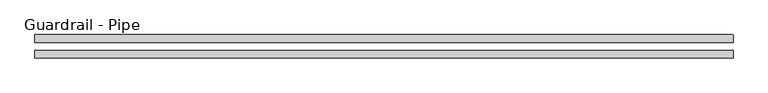
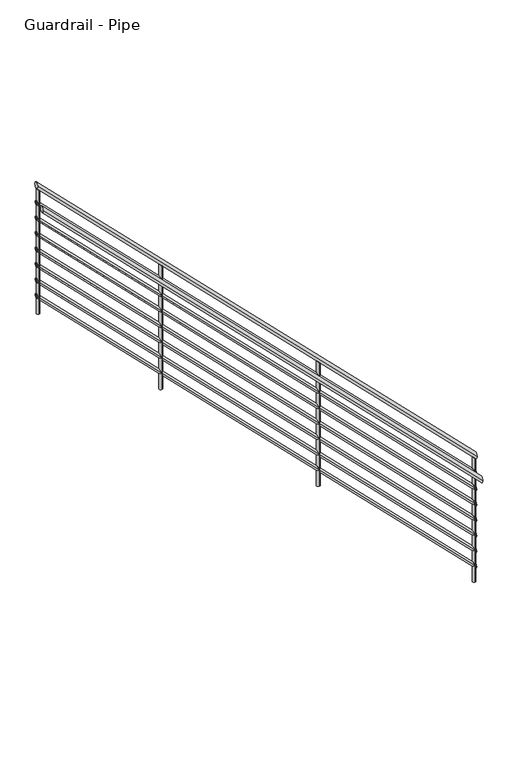
"""IFC4 building model written with IfcOpenShell, lengths in millimetres: railing geometry, Guardrail - Pipe."""

import ifcopenshell
import ifcopenshell.guid

model = None  # the IFC model being written
_history = None  # IfcOwnerHistory: only IFC2X3 demands one
_inside = {}  # id of a spatial element -> (the spatial element, [elements in it])
_under = {}  # id of a project, library or spatial element -> (it, [spatial elements below it])
_declared = {}  # id of a project -> (the project, [libraries it declares])
_typed = {}  # id of a type object -> (the type object, [elements of that type])
_made_of = {}  # id of a material, layer set ... -> (it, [elements and type objects made of it])


def new_model(schema):
    """Start an empty IFC model of exactly this schema.

    Asked for "IFC4X3", IfcOpenShell would pick the latest addendum, in which some entities
    have other attributes; the version numbers below select the first issue.
    IFC2X3 requires an IfcOwnerHistory on every rooted entity: one is made here for all.
    """
    global model, _history
    if schema == "IFC4X3":
        model = ifcopenshell.file(schema_version=(4, 3, 0, 0))
    else:
        model = ifcopenshell.file(schema=schema)
    _inside.clear()
    _under.clear()
    _declared.clear()
    _typed.clear()
    _made_of.clear()
    _history = None
    if model.schema == "IFC2X3":
        org = make("IfcOrganization", Name="unknown")
        user = make(
            "IfcPersonAndOrganization",
            ThePerson=make("IfcPerson", FamilyName="unknown"),
            TheOrganization=org,
        )
        app = make(
            "IfcApplication",
            ApplicationDeveloper=org,
            Version="unknown",
            ApplicationFullName="unknown",
            ApplicationIdentifier="unknown",
        )
        _history = make(
            "IfcOwnerHistory",
            OwningUser=user,
            OwningApplication=app,
            ChangeAction="ADDED",
            CreationDate=0,
        )
    return model


def make(cls, **values):
    """One entity of the class cls with the attributes given. An attribute that is None is left unset."""
    return model.create_entity(
        cls, **{name: value for name, value in values.items() if value is not None}
    )


def rooted(cls, **values):
    """An entity with a GlobalId (a new one), such as an element, a storey or a relation."""
    return make(cls, GlobalId=ifcopenshell.guid.new(), OwnerHistory=_history, **values)


def si_unit(unit_type, name, prefix=None):
    """IfcSIUnit, for example si_unit("LENGTHUNIT", "METRE", prefix="MILLI")."""
    return make("IfcSIUnit", UnitType=unit_type, Prefix=prefix, Name=name)


def assignment(units):
    """IfcUnitAssignment: the units of a project."""
    return None if units is None else make("IfcUnitAssignment", Units=units)


def point(xyz):
    """IfcCartesianPoint."""
    return None if xyz is None else make("IfcCartesianPoint", Coordinates=xyz)


def direction(xyz):
    """IfcDirection."""
    return None if xyz is None else make("IfcDirection", DirectionRatios=xyz)


def frame(location, z_axis=None, x_axis=None):
    """IfcAxis2Placement3D, a coordinate frame: its origin and axes. An axis left out is left unset."""
    return make(
        "IfcAxis2Placement3D",
        Location=point(location),
        Axis=direction(z_axis),
        RefDirection=direction(x_axis),
    )


def origin():
    """The frame at (0, 0, 0) with its axes left unset."""
    return frame((0.0, 0.0, 0.0))


def place(relative_to, where):
    """IfcLocalPlacement: puts the frame where relative to a parent placement (None: the world)."""
    return make(
        "IfcLocalPlacement", PlacementRelTo=relative_to, RelativePlacement=where
    )


def context(
    kind, dimensions, precision=None, world=None, true_north=None, identifier=None
):
    """IfcGeometricRepresentationContext, for example the 3D "Model" context."""
    return make(
        "IfcGeometricRepresentationContext",
        ContextIdentifier=identifier,
        ContextType=kind,
        CoordinateSpaceDimension=dimensions,
        Precision=precision,
        WorldCoordinateSystem=world,
        TrueNorth=true_north,
    )


def project(units=None, contexts=None):
    """IfcProject with its units and contexts."""
    return rooted(
        "IfcProject",
        Name="project",
        RepresentationContexts=contexts,
        UnitsInContext=assignment(units),
    )


def spatial(cls, under=None, at=None, **own):
    """A site, building, storey or space (cls), placed at a placement, below another one or the project."""
    s = rooted(cls, ObjectPlacement=at, **own)
    if under is not None:
        _under.setdefault(under.id(), (under, []))[1].append(s)
    return s


def circle_curve(where, radius):
    """IfcCircle in the frame where."""
    return make("IfcCircle", Position=where, Radius=radius)


def ellipse_curve(where, semi_axis1, semi_axis2):
    """IfcEllipse in the frame where."""
    return make(
        "IfcEllipse", Position=where, SemiAxis1=semi_axis1, SemiAxis2=semi_axis2
    )


def shape(context_of_items, identifier, shape_type, items):
    """IfcShapeRepresentation: the items that make up one representation, for example the "Body"."""
    return make(
        "IfcShapeRepresentation",
        ContextOfItems=context_of_items,
        RepresentationIdentifier=identifier,
        RepresentationType=shape_type,
        Items=items,
    )


def source(mapping_origin, context_of_items, identifier, shape_type, items):
    """IfcRepresentationMap: a shape defined once, which mapped items show again and again."""
    return make(
        "IfcRepresentationMap",
        MappingOrigin=mapping_origin,
        MappedRepresentation=shape(context_of_items, identifier, shape_type, items),
    )


def transform(
    local_origin,
    x_axis=None,
    y_axis=None,
    z_axis=None,
    scale=None,
    scale2=None,
    scale3=None,
    uniform=True,
):
    """IfcCartesianTransformationOperator3D, or its non-uniform kind. x_axis, y_axis, z_axis: its Axis1, 2, 3."""
    if uniform:
        return make(
            "IfcCartesianTransformationOperator3D",
            Axis1=direction(x_axis),
            Axis2=direction(y_axis),
            LocalOrigin=point(local_origin),
            Scale=scale,
            Axis3=direction(z_axis),
        )
    return make(
        "IfcCartesianTransformationOperator3DnonUniform",
        Axis1=direction(x_axis),
        Axis2=direction(y_axis),
        LocalOrigin=point(local_origin),
        Scale=scale,
        Axis3=direction(z_axis),
        Scale2=scale2,
        Scale3=scale3,
    )


def mapped(mapping_source, mapping_target):
    """IfcMappedItem: shows the shape of a source again, moved by a transform."""
    return make(
        "IfcMappedItem", MappingSource=mapping_source, MappingTarget=mapping_target
    )


def made_of(thing, what):
    """Note that an element or type object is made of a material, layer set ...; save() writes the relation."""
    if what is not None:
        _made_of.setdefault(what.id(), (what, []))[1].append(thing)
    return thing


def element(
    cls,
    number,
    at=None,
    inside=None,
    cuts=None,
    type_object=None,
    material=None,
    context=None,
    identifier="Body",
    shape_type=None,
    held_by="IfcProductDefinitionShape",
    body=None,
    shapes=None,
    **own,
):
    """One element of the class cls, such as IfcWall. Its Tag is "e" and its number.

    at: its placement. inside: the storey or other place that contains it. cuts: it is an
    opening in that element (IfcRelVoidsElement). A single representation is given by context,
    identifier, shape_type and body (its items); several are given by shapes. held_by: the class
    of the entity that holds the representations. save() writes the other relations.
    """
    e = rooted(cls, Tag="e%d" % number, ObjectPlacement=at, **own)
    if body is not None:
        shapes = [shape(context, identifier, shape_type, body)]
    if shapes is not None:
        e.Representation = make(held_by, Representations=shapes)
    if inside is not None:
        _inside.setdefault(inside.id(), (inside, []))[1].append(e)
    if cuts is not None:
        rooted(
            "IfcRelVoidsElement", RelatingBuildingElement=cuts, RelatedOpeningElement=e
        )
    if type_object is not None:
        _typed.setdefault(type_object.id(), (type_object, []))[1].append(e)
    return made_of(e, material)


def aggregate(whole, parts):
    """IfcRelAggregates: a whole, such as a stair, and the parts it consists of."""
    return rooted("IfcRelAggregates", RelatingObject=whole, RelatedObjects=parts)


def save(model, path):
    """Write the relations noted so far, then the file.

    IfcRelAggregates (storeys below a building ...), IfcRelContainedInSpatialStructure (elements
    in a storey), IfcRelDefinesByType, IfcRelAssociatesMaterial and IfcRelDeclares: one each for
    every whole, place, type object, material and project.
    """
    for whole, parts in _under.values():
        aggregate(whole, parts)
    for where, things in _inside.values():
        rooted(
            "IfcRelContainedInSpatialStructure",
            RelatedElements=things,
            RelatingStructure=where,
        )
    for kind, things in _typed.values():
        rooted("IfcRelDefinesByType", RelatedObjects=things, RelatingType=kind)
    for what, things in _made_of.values():
        rooted("IfcRelAssociatesMaterial", RelatedObjects=things, RelatingMaterial=what)
    for by, libraries in _declared.values():
        rooted("IfcRelDeclares", RelatingContext=by, RelatedDefinitions=libraries)
    model.write(path)


def plane_surface(at):
    """IfcPlane: the flat surface through the origin of the frame at, square to its z axis."""
    return make("IfcPlane", Position=at)


def cylinder_surface(at, radius):
    """IfcCylindricalSurface: all points at the distance radius from the z axis of the frame at."""
    return make("IfcCylindricalSurface", Position=at, Radius=radius)


def advanced_brep(points, edges, surfaces, faces):
    """IfcAdvancedBrep: a solid bounded by faces that lie on surfaces and meet in shared edges.

    An edge is (start, end): straight between two places in points (the first is 0);
    or (start, end, curve); or (start, end, curve, False) where it runs against its curve.
    A face is (place in surfaces, loops), or (place, loops, False) where it looks against
    its surface's normal. A loop lists edges by number (the first is 1), with a minus sign
    where the edge is run from its end to its start. The first loop is the outer one.
    """
    corners = [point(p) for p in points]
    vertices = [make("IfcVertexPoint", VertexGeometry=c) for c in corners]
    made = []
    for start, end, *more in edges:
        made.append(
            make(
                "IfcEdgeCurve",
                EdgeStart=vertices[start],
                EdgeEnd=vertices[end],
                EdgeGeometry=more[0] if more else make("IfcPolyline", Points=[corners[start], corners[end]]),
                SameSense=more[1] if len(more) > 1 else True,
            )
        )
    hull = []
    for where, loops, *sense in faces:
        bounds = []
        for j, loop in enumerate(loops):
            ring = [make("IfcOrientedEdge", EdgeElement=made[abs(k) - 1], Orientation=k > 0) for k in loop]
            bounds.append(
                make(
                    "IfcFaceOuterBound" if j == 0 else "IfcFaceBound",
                    Bound=make("IfcEdgeLoop", EdgeList=ring),
                    Orientation=True,
                )
            )
        hull.append(make("IfcAdvancedFace", Bounds=bounds, FaceSurface=surfaces[where], SameSense=sense[0] if sense else True))
    return make("IfcAdvancedBrep", Outer=make("IfcClosedShell", CfsFaces=hull))


def guardrail_pipe_ce189c05(model_context):
    return source(origin(), model_context, "Body", "AdvancedBrep", [
        advanced_brep(
        [(-7243.3085296, -3994.9836772, 1268.4592316), (-7243.3085296, -3956.8836772, 1268.4592316), (-10645.1029016, -3994.9836772, 4670.2536037), (-10645.1029016, -3956.8836772, 4670.2536037)],
        [
            (0, 1, ellipse_curve(frame((-7243.3085296, -3975.9336772, 1268.4592316), z_axis=(1.0, 0.0, 0.0), x_axis=(0.0, 0.0, -1.0)), 26.9407684, 19.05)),
            (1, 0, ellipse_curve(frame((-7243.3085296, -3975.9336772, 1268.4592316), z_axis=(1.0, 0.0, 0.0), x_axis=(0.0, 0.0, -1.0)), 26.9407684, 19.05)),
            (2, 3, ellipse_curve(frame((-10645.1029016, -3975.9336772, 4670.2536037), z_axis=(-1.0, 0.0, 0.0), x_axis=(0.0, 0.0, -1.0)), 26.9407684, 19.05)),
            (3, 2, ellipse_curve(frame((-10645.1029016, -3975.9336772, 4670.2536037), z_axis=(-1.0, 0.0, 0.0), x_axis=(0.0, 0.0, -1.0)), 26.9407684, 19.05)),
            (0, 2),
            (3, 1),
        ],
        [
            plane_surface(frame((-7243.3085296, -3975.9336772, 1295.4), z_axis=(1.0, 0.0, 0.0), x_axis=(0.0, -1.0, 0.0))),
            plane_surface(frame((-10645.1029016, -3975.9336772, 4697.194372), z_axis=(-1.0, 0.0, 0.0), x_axis=(0.0, -1.0, 0.0))),
            cylinder_surface(frame((-7256.7789137, -3975.9336772, 1281.9296158), z_axis=(0.7071067811865476, 0.0, -0.7071067811865476), x_axis=(0.0, 1.0, 0.0)), 19.05),
        ],
        [
            (0, [[1, 2]]),
            (1, [[3, 4]]),
            (2, [[-1, 5, -4, 6]]),
            (2, [[-2, -6, -3, -5]]),
        ],
    ),
        advanced_brep(
        [(-7243.3085296, -3988.6336772, 1125.0394878), (-7243.3085296, -3963.2336772, 1125.0394878), (-10645.1029016, -3988.6336772, 4526.8338598), (-10645.1029016, -3963.2336772, 4526.8338598)],
        [
            (0, 1, ellipse_curve(frame((-7243.3085296, -3975.9336772, 1125.0394878), z_axis=(1.0, 0.0, 0.0), x_axis=(0.0, 0.0, -1.0)), 17.9605122, 12.7)),
            (1, 0, ellipse_curve(frame((-7243.3085296, -3975.9336772, 1125.0394878), z_axis=(1.0, 0.0, 0.0), x_axis=(0.0, 0.0, -1.0)), 17.9605122, 12.7)),
            (2, 3, ellipse_curve(frame((-10645.1029016, -3975.9336772, 4526.8338598), z_axis=(-1.0, 0.0, 0.0), x_axis=(0.0, 0.0, -1.0)), 17.9605122, 12.7)),
            (3, 2, ellipse_curve(frame((-10645.1029016, -3975.9336772, 4526.8338598), z_axis=(-1.0, 0.0, 0.0), x_axis=(0.0, 0.0, -1.0)), 17.9605122, 12.7)),
            (0, 2),
            (3, 1),
        ],
        [
            plane_surface(frame((-7243.3085296, -3975.9336772, 1143.0), z_axis=(1.0, 0.0, 0.0), x_axis=(0.0, -1.0, 0.0))),
            plane_surface(frame((-10645.1029016, -3975.9336772, 4544.794372), z_axis=(-1.0, 0.0, 0.0), x_axis=(0.0, -1.0, 0.0))),
            cylinder_surface(frame((-7252.2887857, -3975.9336772, 1134.0197439), z_axis=(0.7071067811865476, 0.0, -0.7071067811865476), x_axis=(0.0, 1.0, 0.0)), 12.7),
        ],
        [
            (0, [[1, 2]]),
            (1, [[3, 4]]),
            (2, [[-1, 5, -4, 6]]),
            (2, [[-2, -6, -3, -5]]),
        ],
    ),
        advanced_brep(
        [(-7243.3085296, -4071.1836772, 1116.0592316), (-7243.3085296, -4033.0836772, 1116.0592316), (-10645.1029016, -4071.1836772, 4517.8536037), (-10645.1029016, -4033.0836772, 4517.8536037)],
        [
            (0, 1, ellipse_curve(frame((-7243.3085296, -4052.1336772, 1116.0592316), z_axis=(1.0, 0.0, 0.0), x_axis=(0.0, 0.0, -1.0)), 26.9407684, 19.05)),
            (1, 0, ellipse_curve(frame((-7243.3085296, -4052.1336772, 1116.0592316), z_axis=(1.0, 0.0, 0.0), x_axis=(0.0, 0.0, -1.0)), 26.9407684, 19.05)),
            (2, 3, ellipse_curve(frame((-10645.1029016, -4052.1336772, 4517.8536037), z_axis=(-1.0, 0.0, 0.0), x_axis=(0.0, 0.0, -1.0)), 26.9407684, 19.05)),
            (3, 2, ellipse_curve(frame((-10645.1029016, -4052.1336772, 4517.8536037), z_axis=(-1.0, 0.0, 0.0), x_axis=(0.0, 0.0, -1.0)), 26.9407684, 19.05)),
            (0, 2),
            (3, 1),
        ],
        [
            plane_surface(frame((-7243.3085296, -4052.1336772, 1143.0), z_axis=(1.0, 0.0, 0.0), x_axis=(0.0, -1.0, 0.0))),
            plane_surface(frame((-10645.1029016, -4052.1336772, 4544.794372), z_axis=(-1.0, 0.0, 0.0), x_axis=(0.0, -1.0, 0.0))),
            cylinder_surface(frame((-7256.7789137, -4052.1336772, 1129.5296158), z_axis=(0.7071067811865476, 0.0, -0.7071067811865476), x_axis=(0.0, 1.0, 0.0)), 19.05),
        ],
        [
            (0, [[1, 2]]),
            (1, [[3, 4]]),
            (2, [[-1, 5, -4, 6]]),
            (2, [[-2, -6, -3, -5]]),
        ],
    ),
        advanced_brep(
        [(-7243.3085296, -3988.6336772, 998.0394878), (-7243.3085296, -3963.2336772, 998.0394878), (-10645.1029016, -3988.6336772, 4399.8338598), (-10645.1029016, -3963.2336772, 4399.8338598)],
        [
            (0, 1, ellipse_curve(frame((-7243.3085296, -3975.9336772, 998.0394878), z_axis=(1.0, 0.0, 0.0), x_axis=(0.0, 0.0, -1.0)), 17.9605122, 12.7)),
            (1, 0, ellipse_curve(frame((-7243.3085296, -3975.9336772, 998.0394878), z_axis=(1.0, 0.0, 0.0), x_axis=(0.0, 0.0, -1.0)), 17.9605122, 12.7)),
            (2, 3, ellipse_curve(frame((-10645.1029016, -3975.9336772, 4399.8338598), z_axis=(-1.0, 0.0, 0.0), x_axis=(0.0, 0.0, -1.0)), 17.9605122, 12.7)),
            (3, 2, ellipse_curve(frame((-10645.1029016, -3975.9336772, 4399.8338598), z_axis=(-1.0, 0.0, 0.0), x_axis=(0.0, 0.0, -1.0)), 17.9605122, 12.7)),
            (0, 2),
            (3, 1),
        ],
        [
            plane_surface(frame((-7243.3085296, -3975.9336772, 1016.0), z_axis=(1.0, 0.0, 0.0), x_axis=(0.0, -1.0, 0.0))),
            plane_surface(frame((-10645.1029016, -3975.9336772, 4417.794372), z_axis=(-1.0, 0.0, 0.0), x_axis=(0.0, -1.0, 0.0))),
            cylinder_surface(frame((-7252.2887857, -3975.9336772, 1007.0197439), z_axis=(0.7071067811865476, 0.0, -0.7071067811865476), x_axis=(0.0, 1.0, 0.0)), 12.7),
        ],
        [
            (0, [[1, 2]]),
            (1, [[3, 4]]),
            (2, [[-1, 5, -4, 6]]),
            (2, [[-2, -6, -3, -5]]),
        ],
    ),
        advanced_brep(
        [(-7243.3085296, -3988.6336772, 871.0394878), (-7243.3085296, -3963.2336772, 871.0394878), (-10645.1029016, -3988.6336772, 4272.8338598), (-10645.1029016, -3963.2336772, 4272.8338598)],
        [
            (0, 1, ellipse_curve(frame((-7243.3085296, -3975.9336772, 871.0394878), z_axis=(1.0, 0.0, 0.0), x_axis=(0.0, 0.0, -1.0)), 17.9605122, 12.7)),
            (1, 0, ellipse_curve(frame((-7243.3085296, -3975.9336772, 871.0394878), z_axis=(1.0, 0.0, 0.0), x_axis=(0.0, 0.0, -1.0)), 17.9605122, 12.7)),
            (2, 3, ellipse_curve(frame((-10645.1029016, -3975.9336772, 4272.8338598), z_axis=(-1.0, 0.0, 0.0), x_axis=(0.0, 0.0, -1.0)), 17.9605122, 12.7)),
            (3, 2, ellipse_curve(frame((-10645.1029016, -3975.9336772, 4272.8338598), z_axis=(-1.0, 0.0, 0.0), x_axis=(0.0, 0.0, -1.0)), 17.9605122, 12.7)),
            (0, 2),
            (3, 1),
        ],
        [
            plane_surface(frame((-7243.3085296, -3975.9336772, 889.0), z_axis=(1.0, 0.0, 0.0), x_axis=(0.0, -1.0, 0.0))),
            plane_surface(frame((-10645.1029016, -3975.9336772, 4290.794372), z_axis=(-1.0, 0.0, 0.0), x_axis=(0.0, -1.0, 0.0))),
            cylinder_surface(frame((-7252.2887857, -3975.9336772, 880.0197439), z_axis=(0.7071067811865476, 0.0, -0.7071067811865476), x_axis=(0.0, 1.0, 0.0)), 12.7),
        ],
        [
            (0, [[1, 2]]),
            (1, [[3, 4]]),
            (2, [[-1, 5, -4, 6]]),
            (2, [[-2, -6, -3, -5]]),
        ],
    ),
        advanced_brep(
        [(-7243.3085296, -3988.6336772, 744.0394878), (-7243.3085296, -3963.2336772, 744.0394878), (-10645.1029016, -3988.6336772, 4145.8338598), (-10645.1029016, -3963.2336772, 4145.8338598)],
        [
            (0, 1, ellipse_curve(frame((-7243.3085296, -3975.9336772, 744.0394878), z_axis=(1.0, 0.0, 0.0), x_axis=(0.0, 0.0, -1.0)), 17.9605122, 12.7)),
            (1, 0, ellipse_curve(frame((-7243.3085296, -3975.9336772, 744.0394878), z_axis=(1.0, 0.0, 0.0), x_axis=(0.0, 0.0, -1.0)), 17.9605122, 12.7)),
            (2, 3, ellipse_curve(frame((-10645.1029016, -3975.9336772, 4145.8338598), z_axis=(-1.0, 0.0, 0.0), x_axis=(0.0, 0.0, -1.0)), 17.9605122, 12.7)),
            (3, 2, ellipse_curve(frame((-10645.1029016, -3975.9336772, 4145.8338598), z_axis=(-1.0, 0.0, 0.0), x_axis=(0.0, 0.0, -1.0)), 17.9605122, 12.7)),
            (0, 2),
            (3, 1),
        ],
        [
            plane_surface(frame((-7243.3085296, -3975.9336772, 762.0), z_axis=(1.0, 0.0, 0.0), x_axis=(0.0, -1.0, 0.0))),
            plane_surface(frame((-10645.1029016, -3975.9336772, 4163.794372), z_axis=(-1.0, 0.0, 0.0), x_axis=(0.0, -1.0, 0.0))),
            cylinder_surface(frame((-7252.2887857, -3975.9336772, 753.0197439), z_axis=(0.7071067811865476, 0.0, -0.7071067811865476), x_axis=(0.0, 1.0, 0.0)), 12.7),
        ],
        [
            (0, [[1, 2]]),
            (1, [[3, 4]]),
            (2, [[-1, 5, -4, 6]]),
            (2, [[-2, -6, -3, -5]]),
        ],
    ),
        advanced_brep(
        [(-7243.3085296, -3988.6336772, 617.0394878), (-7243.3085296, -3963.2336772, 617.0394878), (-10645.1029016, -3988.6336772, 4018.8338598), (-10645.1029016, -3963.2336772, 4018.8338598)],
        [
            (0, 1, ellipse_curve(frame((-7243.3085296, -3975.9336772, 617.0394878), z_axis=(1.0, 0.0, 0.0), x_axis=(0.0, 0.0, -1.0)), 17.9605122, 12.7)),
            (1, 0, ellipse_curve(frame((-7243.3085296, -3975.9336772, 617.0394878), z_axis=(1.0, 0.0, 0.0), x_axis=(0.0, 0.0, -1.0)), 17.9605122, 12.7)),
            (2, 3, ellipse_curve(frame((-10645.1029016, -3975.9336772, 4018.8338598), z_axis=(-1.0, 0.0, 0.0), x_axis=(0.0, 0.0, -1.0)), 17.9605122, 12.7)),
            (3, 2, ellipse_curve(frame((-10645.1029016, -3975.9336772, 4018.8338598), z_axis=(-1.0, 0.0, 0.0), x_axis=(0.0, 0.0, -1.0)), 17.9605122, 12.7)),
            (0, 2),
            (3, 1),
        ],
        [
            plane_surface(frame((-7243.3085296, -3975.9336772, 635.0), z_axis=(1.0, 0.0, 0.0), x_axis=(0.0, -1.0, 0.0))),
            plane_surface(frame((-10645.1029016, -3975.9336772, 4036.794372), z_axis=(-1.0, 0.0, 0.0), x_axis=(0.0, -1.0, 0.0))),
            cylinder_surface(frame((-7252.2887857, -3975.9336772, 626.0197439), z_axis=(0.7071067811865476, 0.0, -0.7071067811865476), x_axis=(0.0, 1.0, 0.0)), 12.7),
        ],
        [
            (0, [[1, 2]]),
            (1, [[3, 4]]),
            (2, [[-1, 5, -4, 6]]),
            (2, [[-2, -6, -3, -5]]),
        ],
    ),
        advanced_brep(
        [(-7243.3085296, -3988.6336772, 490.0394878), (-7243.3085296, -3963.2336772, 490.0394878), (-10645.1029016, -3988.6336772, 3891.8338598), (-10645.1029016, -3963.2336772, 3891.8338598)],
        [
            (0, 1, ellipse_curve(frame((-7243.3085296, -3975.9336772, 490.0394878), z_axis=(1.0, 0.0, 0.0), x_axis=(0.0, 0.0, -1.0)), 17.9605122, 12.7)),
            (1, 0, ellipse_curve(frame((-7243.3085296, -3975.9336772, 490.0394878), z_axis=(1.0, 0.0, 0.0), x_axis=(0.0, 0.0, -1.0)), 17.9605122, 12.7)),
            (2, 3, ellipse_curve(frame((-10645.1029016, -3975.9336772, 3891.8338598), z_axis=(-1.0, 0.0, 0.0), x_axis=(0.0, 0.0, -1.0)), 17.9605122, 12.7)),
            (3, 2, ellipse_curve(frame((-10645.1029016, -3975.9336772, 3891.8338598), z_axis=(-1.0, 0.0, 0.0), x_axis=(0.0, 0.0, -1.0)), 17.9605122, 12.7)),
            (0, 2),
            (3, 1),
        ],
        [
            plane_surface(frame((-7243.3085296, -3975.9336772, 508.0), z_axis=(1.0, 0.0, 0.0), x_axis=(0.0, -1.0, 0.0))),
            plane_surface(frame((-10645.1029016, -3975.9336772, 3909.794372), z_axis=(-1.0, 0.0, 0.0), x_axis=(0.0, -1.0, 0.0))),
            cylinder_surface(frame((-7252.2887857, -3975.9336772, 499.0197439), z_axis=(0.7071067811865476, 0.0, -0.7071067811865476), x_axis=(0.0, 1.0, 0.0)), 12.7),
        ],
        [
            (0, [[1, 2]]),
            (1, [[3, 4]]),
            (2, [[-1, 5, -4, 6]]),
            (2, [[-2, -6, -3, -5]]),
        ],
    ),
        advanced_brep(
        [(-7243.3085296, -3988.6336772, 363.0394878), (-7243.3085296, -3963.2336772, 363.0394878), (-10645.1029016, -3988.6336772, 3764.8338598), (-10645.1029016, -3963.2336772, 3764.8338598)],
        [
            (0, 1, ellipse_curve(frame((-7243.3085296, -3975.9336772, 363.0394878), z_axis=(1.0, 0.0, 0.0), x_axis=(0.0, 0.0, -1.0)), 17.9605122, 12.7)),
            (1, 0, ellipse_curve(frame((-7243.3085296, -3975.9336772, 363.0394878), z_axis=(1.0, 0.0, 0.0), x_axis=(0.0, 0.0, -1.0)), 17.9605122, 12.7)),
            (2, 3, ellipse_curve(frame((-10645.1029016, -3975.9336772, 3764.8338598), z_axis=(-1.0, 0.0, 0.0), x_axis=(0.0, 0.0, -1.0)), 17.9605122, 12.7)),
            (3, 2, ellipse_curve(frame((-10645.1029016, -3975.9336772, 3764.8338598), z_axis=(-1.0, 0.0, 0.0), x_axis=(0.0, 0.0, -1.0)), 17.9605122, 12.7)),
            (0, 2),
            (3, 1),
        ],
        [
            plane_surface(frame((-7243.3085296, -3975.9336772, 381.0), z_axis=(1.0, 0.0, 0.0), x_axis=(0.0, -1.0, 0.0))),
            plane_surface(frame((-10645.1029016, -3975.9336772, 3782.794372), z_axis=(-1.0, 0.0, 0.0), x_axis=(0.0, -1.0, 0.0))),
            cylinder_surface(frame((-7252.2887857, -3975.9336772, 372.0197439), z_axis=(0.7071067811865476, 0.0, -0.7071067811865476), x_axis=(0.0, 1.0, 0.0)), 12.7),
        ],
        [
            (0, [[1, 2]]),
            (1, [[3, 4]]),
            (2, [[-1, 5, -4, 6]]),
            (2, [[-2, -6, -3, -5]]),
        ],
    ),
        advanced_brep(
        [(-9681.7085296, -3963.2336772, 3679.9184633), (-9681.7085296, -3963.2336772, 2667.0), (-9681.7085296, -3988.6336772, 2667.0), (-9681.7085296, -3988.6336772, 3679.9184633)],
        [
            (0, 1),
            (1, 2, circle_curve(frame((-9681.7085296, -3975.9336772, 2667.0), z_axis=(0.0, 0.0, 1.0), x_axis=(0.0, -1.0, 0.0)), 12.7)),
            (2, 3),
            (3, 0, ellipse_curve(frame((-9681.7085296, -3975.9336772, 3679.9184633), z_axis=(-0.7071067811865471, 0.0, -0.7071067811865479), x_axis=(-0.7071067811865479, 0.0, 0.7071067811865471)), 17.9605122, 12.7)),
            (0, 3, ellipse_curve(frame((-9681.7085296, -3975.9336772, 3679.9184633), z_axis=(-0.7071067811865471, 0.0, -0.7071067811865479), x_axis=(-0.7071067811865479, 0.0, 0.7071067811865471)), 17.9605122, 12.7)),
            (2, 1, circle_curve(frame((-9681.7085296, -3975.9336772, 2667.0), z_axis=(0.0, 0.0, 1.0), x_axis=(0.0, -1.0, 0.0)), 12.7)),
        ],
        [
            cylinder_surface(frame((-9681.7085296, -3975.9336772, 2438.4), z_axis=(0.0, 0.0, 1.0), x_axis=(0.0, -1.0, 0.0)), 12.7),
            plane_surface(frame((-9707.1085296, -4001.3336772, 3705.3184633), z_axis=(0.7071067811865471, 0.0, 0.7071067811865479), x_axis=(0.0, 1.0, 0.0))),
            plane_surface(frame((-9656.3085296, -4001.3336772, 2667.0), z_axis=(0.0, 0.0, -1.0), x_axis=(0.0, 1.0, 0.0))),
        ],
        [
            (0, [[1, 2, 3, 4]]),
            (0, [[-1, 5, -3, 6]]),
            (1, [[-4, -5]]),
            (2, [[-2, -6]]),
        ],
    ),
        advanced_brep(
        [(-8462.5085296, -3963.2336772, 2460.7184633), (-8462.5085296, -3963.2336772, 1447.8), (-8462.5085296, -3988.6336772, 1447.8), (-8462.5085296, -3988.6336772, 2460.7184633)],
        [
            (0, 1),
            (1, 2, circle_curve(frame((-8462.5085296, -3975.9336772, 1447.8), z_axis=(0.0, 0.0, 1.0), x_axis=(0.0, -1.0, 0.0)), 12.7)),
            (2, 3),
            (3, 0, ellipse_curve(frame((-8462.5085296, -3975.9336772, 2460.7184633), z_axis=(-0.7071067811865471, 0.0, -0.7071067811865479), x_axis=(-0.7071067811865479, 0.0, 0.7071067811865471)), 17.9605122, 12.7)),
            (0, 3, ellipse_curve(frame((-8462.5085296, -3975.9336772, 2460.7184633), z_axis=(-0.7071067811865471, 0.0, -0.7071067811865479), x_axis=(-0.7071067811865479, 0.0, 0.7071067811865471)), 17.9605122, 12.7)),
            (2, 1, circle_curve(frame((-8462.5085296, -3975.9336772, 1447.8), z_axis=(0.0, 0.0, 1.0), x_axis=(0.0, -1.0, 0.0)), 12.7)),
        ],
        [
            cylinder_surface(frame((-8462.5085296, -3975.9336772, 1219.2), z_axis=(0.0, 0.0, 1.0), x_axis=(0.0, -1.0, 0.0)), 12.7),
            plane_surface(frame((-8487.9085296, -4001.3336772, 2486.1184633), z_axis=(0.7071067811865471, 0.0, 0.7071067811865479), x_axis=(0.0, 1.0, 0.0))),
            plane_surface(frame((-8437.1085296, -4001.3336772, 1447.8), z_axis=(0.0, 0.0, -1.0), x_axis=(0.0, 1.0, 0.0))),
        ],
        [
            (0, [[1, 2, 3, 4]]),
            (0, [[-1, 5, -3, 6]]),
            (1, [[-4, -5]]),
            (2, [[-2, -6]]),
        ],
    ),
        advanced_brep(
        [(-10632.4029016, -3963.2336772, 4630.6128353), (-10632.4029016, -3963.2336772, 3617.694372), (-10632.4029016, -3988.6336772, 3617.694372), (-10632.4029016, -3988.6336772, 4630.6128353)],
        [
            (0, 1),
            (1, 2, circle_curve(frame((-10632.4029016, -3975.9336772, 3617.694372), z_axis=(0.0, 0.0, 1.0), x_axis=(0.0, -1.0, 0.0)), 12.7)),
            (2, 3),
            (3, 0, ellipse_curve(frame((-10632.4029016, -3975.9336772, 4630.6128353), z_axis=(-0.7071067811865471, 0.0, -0.7071067811865479), x_axis=(-0.7071067811865479, 0.0, 0.7071067811865471)), 17.9605122, 12.7)),
            (0, 3, ellipse_curve(frame((-10632.4029016, -3975.9336772, 4630.6128353), z_axis=(-0.7071067811865471, 0.0, -0.7071067811865479), x_axis=(-0.7071067811865479, 0.0, 0.7071067811865471)), 17.9605122, 12.7)),
            (2, 1, circle_curve(frame((-10632.4029016, -3975.9336772, 3617.694372), z_axis=(0.0, 0.0, 1.0), x_axis=(0.0, -1.0, 0.0)), 12.7)),
        ],
        [
            cylinder_surface(frame((-10632.4029016, -3975.9336772, 3389.094372), z_axis=(0.0, 0.0, 1.0), x_axis=(0.0, -1.0, 0.0)), 12.7),
            plane_surface(frame((-10657.8029016, -4001.3336772, 4656.0128353), z_axis=(0.7071067811865471, 0.0, 0.7071067811865479), x_axis=(0.0, 1.0, 0.0))),
            plane_surface(frame((-10607.0029016, -4001.3336772, 3617.694372), z_axis=(0.0, 0.0, -1.0), x_axis=(0.0, 1.0, 0.0))),
        ],
        [
            (0, [[1, 2, 3, 4]]),
            (0, [[-1, 5, -3, 6]]),
            (1, [[-4, -5]]),
            (2, [[-2, -6]]),
        ],
    ),
        advanced_brep(
        [(-7256.0085296, -3963.2336772, 1254.2184633), (-7256.0085296, -3963.2336772, 241.3), (-7256.0085296, -3988.6336772, 241.3), (-7256.0085296, -3988.6336772, 1254.2184633)],
        [
            (0, 1),
            (1, 2, circle_curve(frame((-7256.0085296, -3975.9336772, 241.3), z_axis=(0.0, 0.0, 1.0), x_axis=(0.0, -1.0, 0.0)), 12.7)),
            (2, 3),
            (3, 0, ellipse_curve(frame((-7256.0085296, -3975.9336772, 1254.2184633), z_axis=(-0.7071067811865471, 0.0, -0.7071067811865479), x_axis=(-0.7071067811865479, 0.0, 0.7071067811865471)), 17.9605122, 12.7)),
            (0, 3, ellipse_curve(frame((-7256.0085296, -3975.9336772, 1254.2184633), z_axis=(-0.7071067811865471, 0.0, -0.7071067811865479), x_axis=(-0.7071067811865479, 0.0, 0.7071067811865471)), 17.9605122, 12.7)),
            (2, 1, circle_curve(frame((-7256.0085296, -3975.9336772, 241.3), z_axis=(0.0, 0.0, 1.0), x_axis=(0.0, -1.0, 0.0)), 12.7)),
        ],
        [
            cylinder_surface(frame((-7256.0085296, -3975.9336772, 12.7), z_axis=(0.0, 0.0, 1.0), x_axis=(0.0, -1.0, 0.0)), 12.7),
            plane_surface(frame((-7281.4085296, -4001.3336772, 1279.6184633), z_axis=(0.7071067811865471, 0.0, 0.7071067811865479), x_axis=(0.0, 1.0, 0.0))),
            plane_surface(frame((-7230.6085296, -4001.3336772, 241.3), z_axis=(0.0, 0.0, -1.0), x_axis=(0.0, 1.0, 0.0))),
        ],
        [
            (0, [[1, 2, 3, 4]]),
            (0, [[-1, 5, -3, 6]]),
            (1, [[-4, -5]]),
            (2, [[-2, -6]]),
        ],
    ),
    ])


if __name__ == "__main__":
    model = new_model("IFC4")
    model_context = context("Model", 3, world=origin())
    ifc_project = project(units=[si_unit("LENGTHUNIT", "METRE", prefix="MILLI")], contexts=[model_context])
    site = spatial("IfcSite", under=ifc_project)
    building = spatial("IfcBuilding", under=site)
    placement = place(None, origin())
    guardrail_pipe_shape = guardrail_pipe_ce189c05(model_context)
    element("IfcRailing", 1, ObjectType="Guardrail - Pipe", at=placement, inside=building, context=model_context, shape_type="MappedRepresentation", body=[
        mapped(guardrail_pipe_shape, transform((0.0, 0.0, 0.0), x_axis=(1.0, 0.0, 0.0), y_axis=(0.0, 1.0, 0.0), z_axis=(0.0, 0.0, 1.0))),
    ])
    save(model, "model.ifc")

# Revit data of these elements
# Element 1 (IfcRailing, "Guardrail - Pipe")
#   Materials on its faces: "Plastic - Vinyl Cove Base"
# Materials
#   "Plastic - Vinyl Cove Base": class "Plastic", colour RGB 5 5 5, transparency 0, Cost = 0
